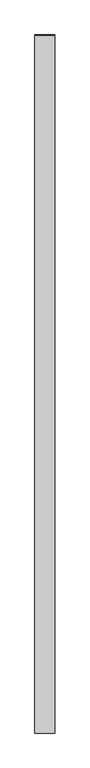
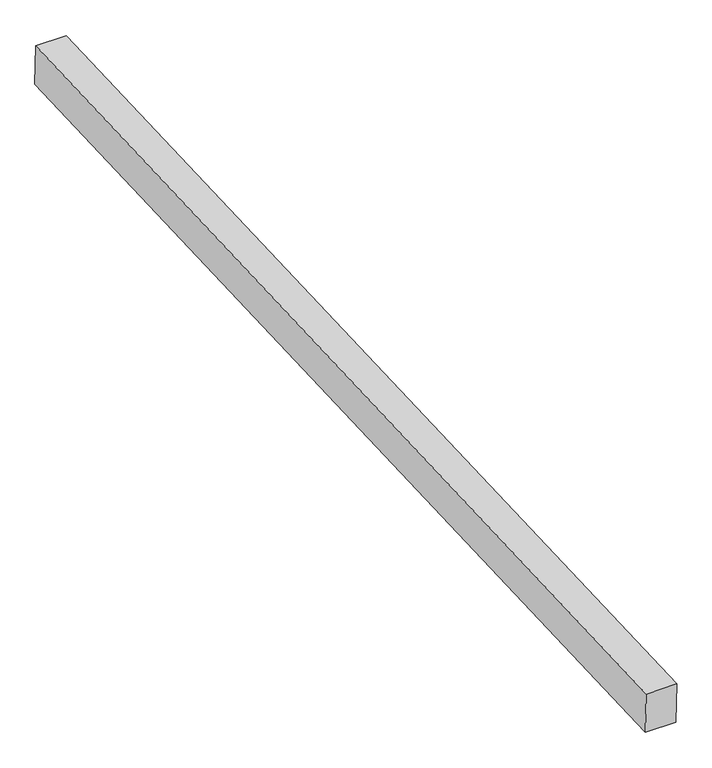
"""IFC4 building model written with IfcOpenShell, lengths in millimetres: proxy geometry, Generic Models 7:Generic Models 1:8:Generic Models 1:8 : Generic Models 7:Generic Models 1:337419:3 : Generic Models 7:Generic Models 1:8:Generic Models 1:8 : Generic Models 7:Generic Models 1:337419:315935."""

import ifcopenshell
import ifcopenshell.guid

model = None  # the IFC model being written
_history = None  # IfcOwnerHistory: only IFC2X3 demands one
_inside = {}  # id of a spatial element -> (the spatial element, [elements in it])
_under = {}  # id of a project, library or spatial element -> (it, [spatial elements below it])
_declared = {}  # id of a project -> (the project, [libraries it declares])
_typed = {}  # id of a type object -> (the type object, [elements of that type])
_made_of = {}  # id of a material, layer set ... -> (it, [elements and type objects made of it])


def new_model(schema):
    """Start an empty IFC model of exactly this schema.

    Asked for "IFC4X3", IfcOpenShell would pick the latest addendum, in which some entities
    have other attributes; the version numbers below select the first issue.
    IFC2X3 requires an IfcOwnerHistory on every rooted entity: one is made here for all.
    """
    global model, _history
    if schema == "IFC4X3":
        model = ifcopenshell.file(schema_version=(4, 3, 0, 0))
    else:
        model = ifcopenshell.file(schema=schema)
    _inside.clear()
    _under.clear()
    _declared.clear()
    _typed.clear()
    _made_of.clear()
    _history = None
    if model.schema == "IFC2X3":
        org = make("IfcOrganization", Name="unknown")
        user = make(
            "IfcPersonAndOrganization",
            ThePerson=make("IfcPerson", FamilyName="unknown"),
            TheOrganization=org,
        )
        app = make(
            "IfcApplication",
            ApplicationDeveloper=org,
            Version="unknown",
            ApplicationFullName="unknown",
            ApplicationIdentifier="unknown",
        )
        _history = make(
            "IfcOwnerHistory",
            OwningUser=user,
            OwningApplication=app,
            ChangeAction="ADDED",
            CreationDate=0,
        )
    return model


def make(cls, **values):
    """One entity of the class cls with the attributes given. An attribute that is None is left unset."""
    return model.create_entity(
        cls, **{name: value for name, value in values.items() if value is not None}
    )


def rooted(cls, **values):
    """An entity with a GlobalId (a new one), such as an element, a storey or a relation."""
    return make(cls, GlobalId=ifcopenshell.guid.new(), OwnerHistory=_history, **values)


def si_unit(unit_type, name, prefix=None):
    """IfcSIUnit, for example si_unit("LENGTHUNIT", "METRE", prefix="MILLI")."""
    return make("IfcSIUnit", UnitType=unit_type, Prefix=prefix, Name=name)


def assignment(units):
    """IfcUnitAssignment: the units of a project."""
    return None if units is None else make("IfcUnitAssignment", Units=units)


def point(xyz):
    """IfcCartesianPoint."""
    return None if xyz is None else make("IfcCartesianPoint", Coordinates=xyz)


def direction(xyz):
    """IfcDirection."""
    return None if xyz is None else make("IfcDirection", DirectionRatios=xyz)


def frame(location, z_axis=None, x_axis=None):
    """IfcAxis2Placement3D, a coordinate frame: its origin and axes. An axis left out is left unset."""
    return make(
        "IfcAxis2Placement3D",
        Location=point(location),
        Axis=direction(z_axis),
        RefDirection=direction(x_axis),
    )


def origin():
    """The frame at (0, 0, 0) with its axes left unset."""
    return frame((0.0, 0.0, 0.0))


def place(relative_to, where):
    """IfcLocalPlacement: puts the frame where relative to a parent placement (None: the world)."""
    return make(
        "IfcLocalPlacement", PlacementRelTo=relative_to, RelativePlacement=where
    )


def context(
    kind, dimensions, precision=None, world=None, true_north=None, identifier=None
):
    """IfcGeometricRepresentationContext, for example the 3D "Model" context."""
    return make(
        "IfcGeometricRepresentationContext",
        ContextIdentifier=identifier,
        ContextType=kind,
        CoordinateSpaceDimension=dimensions,
        Precision=precision,
        WorldCoordinateSystem=world,
        TrueNorth=true_north,
    )


def project(units=None, contexts=None):
    """IfcProject with its units and contexts."""
    return rooted(
        "IfcProject",
        Name="project",
        RepresentationContexts=contexts,
        UnitsInContext=assignment(units),
    )


def spatial(cls, under=None, at=None, **own):
    """A site, building, storey or space (cls), placed at a placement, below another one or the project."""
    s = rooted(cls, ObjectPlacement=at, **own)
    if under is not None:
        _under.setdefault(under.id(), (under, []))[1].append(s)
    return s


def polyline(points):
    """IfcPolyline through the points."""
    return make("IfcPolyline", Points=[point(p) for p in points])


def outline(outer, holes=None, kind="AREA"):
    """IfcArbitraryClosedProfileDef: a profile drawn as a closed curve; with holes, ...WithVoids."""
    if holes is None:
        return make("IfcArbitraryClosedProfileDef", ProfileType=kind, OuterCurve=outer)
    return make(
        "IfcArbitraryProfileDefWithVoids",
        ProfileType=kind,
        OuterCurve=outer,
        InnerCurves=holes,
    )


def extrude(swept, where, along, depth):
    """IfcExtrudedAreaSolid: the profile swept, set in the frame where, extruded along a direction by depth."""
    return make(
        "IfcExtrudedAreaSolid",
        SweptArea=swept,
        Position=where,
        ExtrudedDirection=direction(along),
        Depth=depth,
    )


def shape(context_of_items, identifier, shape_type, items):
    """IfcShapeRepresentation: the items that make up one representation, for example the "Body"."""
    return make(
        "IfcShapeRepresentation",
        ContextOfItems=context_of_items,
        RepresentationIdentifier=identifier,
        RepresentationType=shape_type,
        Items=items,
    )


def source(mapping_origin, context_of_items, identifier, shape_type, items):
    """IfcRepresentationMap: a shape defined once, which mapped items show again and again."""
    return make(
        "IfcRepresentationMap",
        MappingOrigin=mapping_origin,
        MappedRepresentation=shape(context_of_items, identifier, shape_type, items),
    )


def transform(
    local_origin,
    x_axis=None,
    y_axis=None,
    z_axis=None,
    scale=None,
    scale2=None,
    scale3=None,
    uniform=True,
):
    """IfcCartesianTransformationOperator3D, or its non-uniform kind. x_axis, y_axis, z_axis: its Axis1, 2, 3."""
    if uniform:
        return make(
            "IfcCartesianTransformationOperator3D",
            Axis1=direction(x_axis),
            Axis2=direction(y_axis),
            LocalOrigin=point(local_origin),
            Scale=scale,
            Axis3=direction(z_axis),
        )
    return make(
        "IfcCartesianTransformationOperator3DnonUniform",
        Axis1=direction(x_axis),
        Axis2=direction(y_axis),
        LocalOrigin=point(local_origin),
        Scale=scale,
        Axis3=direction(z_axis),
        Scale2=scale2,
        Scale3=scale3,
    )


def mapped(mapping_source, mapping_target):
    """IfcMappedItem: shows the shape of a source again, moved by a transform."""
    return make(
        "IfcMappedItem", MappingSource=mapping_source, MappingTarget=mapping_target
    )


def made_of(thing, what):
    """Note that an element or type object is made of a material, layer set ...; save() writes the relation."""
    if what is not None:
        _made_of.setdefault(what.id(), (what, []))[1].append(thing)
    return thing


def element(
    cls,
    number,
    at=None,
    inside=None,
    cuts=None,
    type_object=None,
    material=None,
    context=None,
    identifier="Body",
    shape_type=None,
    held_by="IfcProductDefinitionShape",
    body=None,
    shapes=None,
    **own,
):
    """One element of the class cls, such as IfcWall. Its Tag is "e" and its number.

    at: its placement. inside: the storey or other place that contains it. cuts: it is an
    opening in that element (IfcRelVoidsElement). A single representation is given by context,
    identifier, shape_type and body (its items); several are given by shapes. held_by: the class
    of the entity that holds the representations. save() writes the other relations.
    """
    e = rooted(cls, Tag="e%d" % number, ObjectPlacement=at, **own)
    if body is not None:
        shapes = [shape(context, identifier, shape_type, body)]
    if shapes is not None:
        e.Representation = make(held_by, Representations=shapes)
    if inside is not None:
        _inside.setdefault(inside.id(), (inside, []))[1].append(e)
    if cuts is not None:
        rooted(
            "IfcRelVoidsElement", RelatingBuildingElement=cuts, RelatedOpeningElement=e
        )
    if type_object is not None:
        _typed.setdefault(type_object.id(), (type_object, []))[1].append(e)
    return made_of(e, material)


def aggregate(whole, parts):
    """IfcRelAggregates: a whole, such as a stair, and the parts it consists of."""
    return rooted("IfcRelAggregates", RelatingObject=whole, RelatedObjects=parts)


def save(model, path):
    """Write the relations noted so far, then the file.

    IfcRelAggregates (storeys below a building ...), IfcRelContainedInSpatialStructure (elements
    in a storey), IfcRelDefinesByType, IfcRelAssociatesMaterial and IfcRelDeclares: one each for
    every whole, place, type object, material and project.
    """
    for whole, parts in _under.values():
        aggregate(whole, parts)
    for where, things in _inside.values():
        rooted(
            "IfcRelContainedInSpatialStructure",
            RelatedElements=things,
            RelatingStructure=where,
        )
    for kind, things in _typed.values():
        rooted("IfcRelDefinesByType", RelatedObjects=things, RelatingType=kind)
    for what, things in _made_of.values():
        rooted("IfcRelAssociatesMaterial", RelatedObjects=things, RelatingMaterial=what)
    for by, libraries in _declared.values():
        rooted("IfcRelDeclares", RelatingContext=by, RelatedDefinitions=libraries)
    model.write(path)


def generic_models_c018e478(model_context):
    return source(origin(), model_context, "Body", "SweptSolid", [
        extrude(outline(polyline([(-580626.555738, 3844.0209448), (-575753.6328438, 4047.0593987), (-575746.0659221, 3856.7093942), (-580618.6251193, 3653.6860944), (-580626.555738, 3844.0209448)])), frame((594890.611724, 0.0, 0.0), z_axis=(1.0, 0.0, 0.0), x_axis=(0.0, 1.0, 0.0)), (0.0, 0.0, 1.0), 139.7),
    ])


if __name__ == "__main__":
    model = new_model("IFC4")
    model_context = context("Model", 3, world=origin())
    ifc_project = project(units=[si_unit("LENGTHUNIT", "METRE", prefix="MILLI")], contexts=[model_context])
    site = spatial("IfcSite", under=ifc_project)
    building = spatial("IfcBuilding", under=site)
    placement = place(None, origin())
    generic_models_shape = generic_models_c018e478(model_context)
    element("IfcBuildingElementProxy", 1, Name="Generic Models 7:Generic Models 1:8:Generic Models 1:8 : Generic Models 7:Generic Models 1:337419:3 : Generic Models 7:Generic Models 1:8:Generic Models 1:8 : Generic Models 7:Generic Models 1:337419:315935", ObjectType="Generic Models 7:Generic Models 1:8:Generic Models 1:8 : Generic Models 7:Generic Models 1:337419:3 : Generic Models 7:Generic Models 1:8:Generic Models 1:8 : Generic Models 7:Generic Models 1:337419:315935", at=placement, inside=building, context=model_context, shape_type="MappedRepresentation", body=[
        mapped(generic_models_shape, transform((0.0, 0.0, 0.0), x_axis=(1.0, 0.0, 0.0), y_axis=(0.0, 1.0, 0.0), z_axis=(0.0, 0.0, 1.0))),
    ])
    save(model, "model.ifc")

# Revit data of these elements
# Type "Generic Models 7:Generic Models 1:8:Generic Models 1:8 : Generic Models 7:Generic Models 1:337419:3 : Generic Models 7:Generic Models 1:8:Generic Models 1:8 : Generic Models 7:Generic Models 1:337419:315935"
#   NameOverride = "Generic Models 7:Generic Models 1:8:Generic Models 1:8 : Generic Models 7:Generic Models 1:337419:315935"
#   ObjectTypeOverride = "Generic Models 1:8 : Generic Models 7:Generic Models 1:337419"
#   Reference = "Generic Models 1"
#   Tag = "315935"
# Element 1 (IfcBuildingElementProxy, "Generic Models 7:Generic Models 1:8:Generic Models 1:8 : Generic Models 7:Generic Models 1:337419:3 : Generic Models 7:Generic Models 1:8:Generic Models 1:8 : Generic Models 7:Generic Models 1:337419:315935")
#   Materials on its faces: "5 1/8\" X 7 1/2\" EXTERIOR GRADE GLULAM BEAMS (4'- 0 1/4\" O.C.)"
# Materials
#   "5 1/8\" X 7 1/2\" EXTERIOR GRADE GLULAM BEAMS (4'- 0 1/4\" O.C.)": class "Wood", colour RGB 183 134 68, transparency 0, Keynote = "M06181300.01", Description = "Pinus Echinata", Cost = 0
